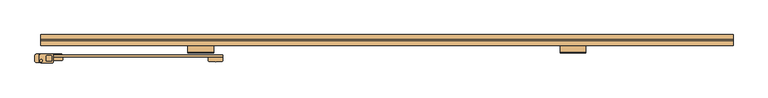
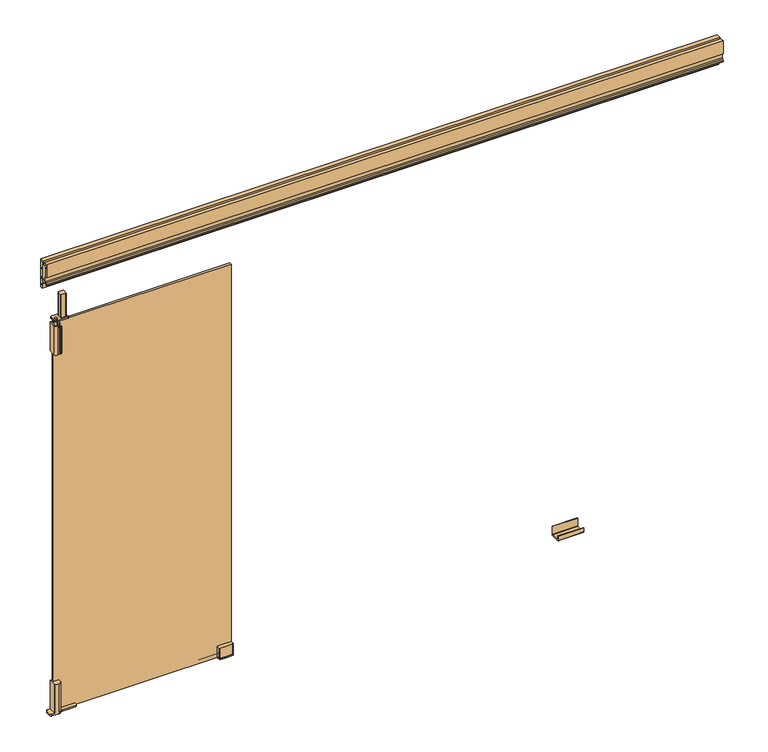
"""IFC4 building model written with IfcOpenShell, lengths in millimetres: door geometry, Otomatik Kapı-Tek Kanat : Otomatik Kapı - Tek Kanat."""

from ifc_helpers import new_model, si_unit, point, frame, frame_2d, origin, origin_with_axes, place, context, project, spatial, polyline, circle_curve, trimmed, segment, composite_curve, outline, extrude, source, transform, mapped, element, save
from ifc_brep_helpers import plane_surface, cylinder_surface, revolved_surface, advanced_brep


def door_8b1a0773(model_context):
    return source(origin(), model_context, "Body", "SolidModel", [
        advanced_brep(
        [(-1574.3473639, -189.1450647, 150.5), (-1574.3473639, -187.0776187, 150.5), (-1576.2799178, -185.1450647, 150.5), (-1605.0612263, -185.1450647, 150.5), (-1606.9937802, -187.0776187, 150.5), (-1606.9937802, -222.3613608, 150.5), (-1605.2100763, -224.1450647, 150.5), (-1587.4005623, -224.1450647, 150.5), (-1574.9937802, -217.3610561, 150.5), (-1574.9937802, -199.1283088, 150.5), (-1599.9937802, -199.1283088, 150.5), (-1599.9937802, -189.1450647, 150.5), (-1578.9203726, -221.1098306, 8.0), (-1577.1630779, -219.3712473, 8.0), (-1574.9937802, -217.3610561, 8.0), (-1599.9937802, -189.1450647, 8.0), (-1574.3473639, -189.1450647, 8.0), (-1599.9937802, -199.1283088, 8.0), (-1574.9937802, -199.1283088, 8.0), (-1587.4005623, -224.1450647, 8.0), (-1605.2100763, -224.1450647, 8.0), (-1619.8416735, -224.1450647, 8.0), (-1619.8416735, -224.1450647, 0.0), (-1587.4005623, -224.1450647, 0.0), (-1606.9937802, -222.3613608, 8.0), (-1606.9937802, -187.0776187, 8.0), (-1605.0612263, -185.1450647, 8.0), (-1576.2799178, -185.1450647, 8.0), (-1504.0, -185.1450647, 8.0), (-1504.0, -185.1450647, 0.0), (-1619.9440671, -185.1450647, 0.0), (-1619.9440671, -185.1450647, 8.0), (-1574.3473639, -187.0776187, 8.0), (-1499.0, -190.1450647, 0.0), (-1499.0, -210.1450647, 0.0), (-1504.0, -215.1450647, 0.0), (-1568.1, -215.1450647, 0.0), (-1577.1630779, -219.3712473, 0.0), (-1627.0, -216.9867382, 0.0), (-1627.0, -192.2009976, 0.0), (-1627.0, -192.2009976, 8.0), (-1627.0, -216.9867382, 8.0), (-1568.1, -215.1450647, 8.0), (-1504.0, -215.1450647, 8.0), (-1499.0, -210.1450647, 8.0), (-1499.0, -190.1450647, 8.0)],
        [
            (0, 1),
            (1, 2, circle_curve(frame((-1576.2799178, -187.0776187, 150.5), z_axis=(0.0, 0.0, 1.0), x_axis=(1.0, 0.0, 0.0)), 1.932554)),
            (2, 3),
            (3, 4, circle_curve(frame((-1605.0612263, -187.0776187, 150.5), z_axis=(0.0, 0.0, 1.0), x_axis=(1.0, 0.0, 0.0)), 1.932554)),
            (4, 5),
            (5, 6, circle_curve(frame((-1605.2100763, -222.3613608, 150.5), z_axis=(0.0, 0.0, 1.0), x_axis=(1.0, 0.0, 0.0)), 1.7837039)),
            (6, 7),
            (7, 8, circle_curve(frame((-1588.8230743, -206.8065986, 150.5), z_axis=(0.0, 0.0, 1.0), x_axis=(1.0, 0.0, 0.0)), 17.3967223)),
            (8, 9),
            (9, 10),
            (10, 11),
            (11, 0),
            (12, 13, circle_curve(frame((-1587.4005623, -210.7809779, 8.0), z_axis=(0.0, 0.0, 1.0), x_axis=(1.0, 0.0, 0.0)), 13.3640868)),
            (13, 14, circle_curve(frame((-1568.1, -226.9760726, 8.0), z_axis=(0.0, 0.0, -1.0), x_axis=(1.0, 0.0, 0.0)), 11.8310079)),
            (14, 12, circle_curve(frame((-1588.8230743, -206.8065986, 8.0), z_axis=(0.0, 0.0, -1.0), x_axis=(1.0, 0.0, 0.0)), 17.3967223)),
            (11, 15),
            (15, 16),
            (16, 0),
            (10, 17),
            (17, 15),
            (9, 18),
            (18, 17),
            (8, 14),
            (14, 18),
            (7, 19),
            (19, 12, circle_curve(frame((-1588.8230743, -206.8065986, 8.0), z_axis=(0.0, 0.0, 1.0), x_axis=(1.0, 0.0, 0.0)), 17.3967223)),
            (6, 20),
            (20, 21),
            (21, 22),
            (22, 23),
            (23, 19),
            (5, 24),
            (24, 20, circle_curve(frame((-1605.2100763, -222.3613608, 8.0), z_axis=(0.0, 0.0, 1.0), x_axis=(1.0, 0.0, 0.0)), 1.7837039)),
            (4, 25),
            (25, 24),
            (3, 26),
            (26, 25, circle_curve(frame((-1605.0612263, -187.0776187, 8.0), z_axis=(0.0, 0.0, 1.0), x_axis=(1.0, 0.0, 0.0)), 1.932554)),
            (2, 27),
            (27, 28),
            (28, 29),
            (29, 30),
            (30, 31),
            (31, 26),
            (1, 32),
            (32, 27, circle_curve(frame((-1576.2799178, -187.0776187, 8.0), z_axis=(0.0, 0.0, 1.0), x_axis=(1.0, 0.0, 0.0)), 1.932554)),
            (16, 32),
            (29, 33, circle_curve(frame((-1504.0, -190.1450647, 0.0), z_axis=(0.0, 0.0, -1.0), x_axis=(1.0, 0.0, 0.0)), 5.0)),
            (33, 34),
            (34, 35, circle_curve(frame((-1504.0, -210.1450647, 0.0), z_axis=(0.0, 0.0, -1.0), x_axis=(1.0, 0.0, 0.0)), 5.0)),
            (35, 36),
            (36, 37, circle_curve(frame((-1568.1, -226.9760726, 0.0), z_axis=(0.0, 0.0, 1.0), x_axis=(1.0, 0.0, 0.0)), 11.8310079)),
            (37, 23, circle_curve(frame((-1587.4005623, -210.7809779, 0.0), z_axis=(0.0, 0.0, -1.0), x_axis=(1.0, 0.0, 0.0)), 13.3640868)),
            (22, 38, circle_curve(frame((-1619.8416735, -216.9867382, 0.0), z_axis=(0.0, 0.0, -1.0), x_axis=(1.0, 0.0, 0.0)), 7.1583265)),
            (38, 39),
            (39, 30, circle_curve(frame((-1619.9440671, -192.2009976, 0.0), z_axis=(0.0, 0.0, -1.0), x_axis=(1.0, 0.0, 0.0)), 7.0559329)),
            (19, 12, circle_curve(frame((-1587.4005623, -210.7809779, 8.0), z_axis=(0.0, 0.0, 1.0), x_axis=(1.0, 0.0, 0.0)), 13.3640868)),
            (31, 40, circle_curve(frame((-1619.9440671, -192.2009976, 8.0), z_axis=(0.0, 0.0, 1.0), x_axis=(1.0, 0.0, 0.0)), 7.0559329)),
            (40, 41),
            (41, 21, circle_curve(frame((-1619.8416735, -216.9867382, 8.0), z_axis=(0.0, 0.0, 1.0), x_axis=(1.0, 0.0, 0.0)), 7.1583265)),
            (14, 42, circle_curve(frame((-1568.1, -226.9760726, 8.0), z_axis=(0.0, 0.0, -1.0), x_axis=(1.0, 0.0, 0.0)), 11.8310079)),
            (42, 43),
            (43, 44, circle_curve(frame((-1504.0, -210.1450647, 8.0), z_axis=(0.0, 0.0, 1.0), x_axis=(1.0, 0.0, 0.0)), 5.0)),
            (44, 45),
            (45, 28, circle_curve(frame((-1504.0, -190.1450647, 8.0), z_axis=(0.0, 0.0, 1.0), x_axis=(1.0, 0.0, 0.0)), 5.0)),
            (39, 40),
            (38, 41),
            (37, 13),
            (36, 42),
            (35, 43),
            (34, 44),
            (33, 45),
        ],
        [
            plane_surface(frame((-1627.0, -185.1450647, 150.5), z_axis=(0.0, 0.0, 1.0), x_axis=(0.0, 1.0, 0.0))),
            plane_surface(frame((-1627.0, -185.1450647, 8.0), z_axis=(0.0, 0.0, -1.0), x_axis=(0.0, 1.0, 0.0))),
            plane_surface(frame((-1574.3473639, -189.1450647, 150.5), z_axis=(0.0, -1.0, 0.0), x_axis=(0.0, 0.0, -1.0))),
            plane_surface(frame((-1599.9937802, -189.1450647, 150.5), z_axis=(1.0, 0.0, 0.0), x_axis=(0.0, 0.0, -1.0))),
            plane_surface(frame((-1599.9937802, -199.1283088, 150.5), z_axis=(0.0, 1.0, 0.0), x_axis=(0.0, 0.0, -1.0))),
            plane_surface(frame((-1574.9937802, -199.1283088, 150.5), z_axis=(1.0, 0.0, 0.0), x_axis=(0.0, 0.0, -1.0))),
            cylinder_surface(frame((-1588.8230743, -206.8065986, 150.5), z_axis=(0.0, 0.0, 1.0), x_axis=(1.0, 0.0, 0.0)), 17.3967223),
            plane_surface(frame((-1587.4005623, -224.1450647, 150.5), z_axis=(0.0, -1.0, 0.0), x_axis=(0.0, 0.0, -1.0))),
            cylinder_surface(frame((-1605.2100763, -222.3613608, 150.5), z_axis=(0.0, 0.0, 1.0), x_axis=(1.0, 0.0, 0.0)), 1.7837039),
            plane_surface(frame((-1606.9937802, -222.3613608, 150.5), z_axis=(-1.0, 0.0, 0.0), x_axis=(0.0, 0.0, -1.0))),
            cylinder_surface(frame((-1605.0612263, -187.0776187, 150.5), z_axis=(0.0, 0.0, 1.0), x_axis=(1.0, 0.0, 0.0)), 1.932554),
            plane_surface(frame((-1605.0612263, -185.1450647, 150.5), z_axis=(0.0, 1.0, 0.0), x_axis=(0.0, 0.0, -1.0))),
            cylinder_surface(frame((-1576.2799178, -187.0776187, 150.5), z_axis=(0.0, 0.0, 1.0), x_axis=(1.0, 0.0, 0.0)), 1.932554),
            plane_surface(frame((-1574.3473639, -187.0776187, 150.5), z_axis=(1.0, 0.0, 0.0), x_axis=(0.0, 0.0, -1.0))),
            plane_surface(frame((-1627.0, -185.1450647, 0.0), z_axis=(0.0, 0.0, -1.0), x_axis=(0.0, 1.0, 0.0))),
            plane_surface(frame((-1627.0, -185.1450647, 8.0), z_axis=(0.0, 0.0, 1.0), x_axis=(0.0, 1.0, 0.0))),
            cylinder_surface(frame((-1619.9440671, -192.2009976, 0.0), z_axis=(0.0, 0.0, -1.0), x_axis=(1.0, 0.0, 0.0)), 7.0559329),
            plane_surface(frame((-1627.0, -192.2009976, 0.0), z_axis=(-1.0, 0.0, 0.0), x_axis=(0.0, 0.0, 1.0))),
            cylinder_surface(frame((-1619.8416735, -216.9867382, 0.0), z_axis=(0.0, 0.0, -1.0), x_axis=(1.0, 0.0, 0.0)), 7.1583265),
            cylinder_surface(frame((-1587.4005623, -210.7809779, 0.0), z_axis=(0.0, 0.0, -1.0), x_axis=(1.0, 0.0, 0.0)), 13.3640868),
            revolved_surface(polyline([(-1556.2689920999999, -226.9760726, 8.0), (-1556.2689920999999, -226.9760726, 0.0)]), (-1568.1, -226.9760726, 0.0), (0.0, 0.0, 1.0)),
            plane_surface(frame((-1568.1, -215.1450647, 0.0), z_axis=(0.0, -1.0, 0.0), x_axis=(0.0, 0.0, 1.0))),
            cylinder_surface(frame((-1504.0, -210.1450647, 0.0), z_axis=(0.0, 0.0, -1.0), x_axis=(1.0, 0.0, 0.0)), 5.0),
            plane_surface(frame((-1499.0, -210.1450647, 0.0), z_axis=(1.0, 0.0, 0.0), x_axis=(0.0, 0.0, 1.0))),
            cylinder_surface(frame((-1504.0, -190.1450647, 0.0), z_axis=(0.0, 0.0, -1.0), x_axis=(1.0, 0.0, 0.0)), 5.0),
        ],
        [
            (0, [[1, 2, 3, 4, 5, 6, 7, 8, 9, 10, 11, 12]]),
            (1, [[13, 14, 15]]),
            (2, [[16, 17, 18, -12]]),
            (3, [[19, 20, -16, -11]]),
            (4, [[21, 22, -19, -10]]),
            (5, [[23, 24, -21, -9]]),
            (6, [[25, 26, -15, -23, -8]]),
            (7, [[27, 28, 29, 30, 31, -25, -7]]),
            (8, [[32, 33, -27, -6]]),
            (9, [[34, 35, -32, -5]]),
            (10, [[36, 37, -34, -4]]),
            (11, [[38, 39, 40, 41, 42, 43, -36, -3]]),
            (12, [[44, 45, -38, -2]]),
            (13, [[-18, 46, -44, -1]]),
            (14, [[47, 48, 49, 50, 51, 52, -30, 53, 54, 55, -41]]),
            (15, [[-26, 56]]),
            (15, [[-28, -33, -35, -37, -43, 57, 58, 59]]),
            (15, [[-39, -45, -46, -17, -20, -22, -24, 60, 61, 62, 63, 64]]),
            (16, [[65, -57, -42, -55]]),
            (17, [[66, -58, -65, -54]]),
            (18, [[-29, -59, -66, -53]]),
            (19, [[67, -13, -56, -31, -52]]),
            (20, [[68, -60, -14, -67, -51]]),
            (21, [[69, -61, -68, -50]]),
            (22, [[70, -62, -69, -49]]),
            (23, [[71, -63, -70, -48]]),
            (24, [[-40, -64, -71, -47]]),
        ],
    ),
        advanced_brep(
        [(-1572.1438552, -192.4241594, 2085.0), (-1573.9791404, -194.2594446, 2085.0), (-1573.9791404, -215.5888742, 2085.0), (-1572.1438552, -217.4241594, 2085.0), (-1550.8144257, -217.4241594, 2085.0), (-1548.9791404, -215.5888742, 2085.0), (-1548.9791404, -194.2594446, 2085.0), (-1550.8144257, -192.4241594, 2085.0), (-1550.8144257, -192.4241594, 1970.0), (-1572.1438552, -192.4241594, 1970.0), (-1548.9791404, -194.2594446, 1970.0), (-1548.9791404, -215.5888742, 1970.0), (-1550.8144257, -217.4241594, 1970.0), (-1572.1438552, -217.4241594, 1970.0), (-1573.9791404, -215.5888742, 1970.0), (-1573.9791404, -194.2594446, 1970.0), (-1545.9964024, -185.1450647, 1970.0), (-1598.1649399, -185.1450647, 1970.0), (-1606.9937802, -193.9739051, 1970.0), (-1606.9937802, -216.1450647, 1970.0), (-1597.9937802, -225.1450647, 1970.0), (-1546.3153559, -225.1450647, 1970.0), (-1542.9937802, -221.823489, 1970.0), (-1542.9937802, -188.1476868, 1970.0), (-1597.9937802, -222.0450647, 1970.0), (-1597.9937802, -210.2450647, 1970.0), (-1545.9964024, -185.1450647, 1964.0), (-1542.9937802, -188.1476868, 1964.0), (-1542.9937802, -221.823489, 1964.0), (-1546.3153559, -225.1450647, 1964.0), (-1597.9937802, -225.1450647, 1964.0), (-1606.9937802, -216.1450647, 1964.0), (-1606.9937802, -193.9739051, 1964.0), (-1598.1649399, -185.1450647, 1964.0), (-1597.9937802, -210.2450647, 1964.0), (-1597.9937802, -222.0450647, 1964.0), (-1606.9937802, -216.1450647, 1798.2), (-1606.9937802, -186.3566653, 1798.2), (-1605.7821796, -185.1450647, 1798.2), (-1576.3197681, -185.1450647, 1798.2), (-1574.9937802, -186.4710526, 1798.2), (-1574.9937802, -189.2450647, 1798.2), (-1599.7937802, -189.2450647, 1798.2), (-1599.7937802, -199.2450647, 1798.2), (-1574.9937802, -199.2450647, 1798.2), (-1574.9937802, -222.0450647, 1798.2), (-1578.0937802, -225.1450647, 1798.2), (-1587.411505, -225.1450647, 1798.2), (-1591.4461955, -222.319944, 1798.2), (-1587.2194224, -210.2450647, 1798.2), (-1588.9937802, -212.0194225, 1798.2), (-1588.9937802, -219.8725331, 1798.2), (-1587.1673699, -222.0450647, 1798.2), (-1579.0825581, -222.0450647, 1798.2), (-1578.0937802, -221.0562868, 1798.2), (-1578.0937802, -210.2450647, 1798.2), (-1597.9937802, -210.2450647, 1798.2), (-1597.9937802, -222.0450647, 1798.2), (-1606.9937802, -216.1450647, 1943.2), (-1588.9937802, -216.1450647, 1943.2), (-1588.9937802, -212.0194225, 1943.2), (-1587.2194224, -210.2450647, 1943.2), (-1576.1717604, -210.2450647, 1943.2), (-1574.9937802, -209.0670845, 1943.2), (-1574.9937802, -199.2450647, 1943.2), (-1599.7937802, -199.2450647, 1943.2), (-1599.7937802, -189.2450647, 1943.2), (-1574.9937802, -189.2450647, 1943.2), (-1574.9937802, -186.4710526, 1943.2), (-1576.3197681, -185.1450647, 1943.2), (-1605.7821796, -185.1450647, 1943.2), (-1606.9937802, -186.3566653, 1943.2), (-1597.9937802, -222.0450647, 1943.2), (-1597.9937802, -210.2450647, 1943.2), (-1574.9937802, -209.0670845, 1933.2), (-1574.9937802, -222.0450647, 1933.2), (-1576.1717604, -210.2450647, 1933.2), (-1578.0937802, -210.2450647, 1933.2), (-1588.9937802, -216.1450647, 1933.2), (-1588.9937802, -219.8725331, 1933.2), (-1591.4461955, -222.319944, 1933.2), (-1597.9937802, -210.2450647, 1943.2), (-1597.9937802, -222.0450647, 1943.2), (-1578.0937802, -225.1450647, 1933.2), (-1578.0937802, -221.0562868, 1933.2), (-1579.0825581, -222.0450647, 1933.2), (-1587.1673699, -222.0450647, 1933.2), (-1587.411505, -225.1450647, 1933.2), (-1597.9937802, -210.2450647, 1976.5286826), (-1597.9937802, -222.0450647, 1976.5286826)],
        [
            (0, 1, circle_curve(frame((-1572.1438552, -194.2594446, 2085.0), z_axis=(0.0, 0.0, 1.0), x_axis=(0.0, -1.0, 0.0)), 1.8352852)),
            (1, 2),
            (2, 3, circle_curve(frame((-1572.1438552, -215.5888742, 2085.0), z_axis=(0.0, 0.0, 1.0), x_axis=(0.0, 1.0, 0.0)), 1.8352852)),
            (3, 4),
            (4, 5, circle_curve(frame((-1550.8144257, -215.5888742, 2085.0), z_axis=(0.0, 0.0, 1.0), x_axis=(0.0, 1.0, 0.0)), 1.8352852)),
            (5, 6),
            (6, 7, circle_curve(frame((-1550.8144257, -194.2594446, 2085.0), z_axis=(0.0, 0.0, 1.0), x_axis=(0.0, -1.0, 0.0)), 1.8352852)),
            (7, 0),
            (7, 8),
            (8, 9),
            (9, 0),
            (6, 10),
            (10, 8, circle_curve(frame((-1550.8144257, -194.2594446, 1970.0), z_axis=(0.0, 0.0, 1.0), x_axis=(0.0, -1.0, 0.0)), 1.8352852)),
            (5, 11),
            (11, 10),
            (4, 12),
            (12, 11, circle_curve(frame((-1550.8144257, -215.5888742, 1970.0), z_axis=(0.0, 0.0, 1.0), x_axis=(0.0, 1.0, 0.0)), 1.8352852)),
            (3, 13),
            (13, 12),
            (2, 14),
            (14, 13, circle_curve(frame((-1572.1438552, -215.5888742, 1970.0), z_axis=(0.0, 0.0, 1.0), x_axis=(0.0, 1.0, 0.0)), 1.8352852)),
            (1, 15),
            (15, 14),
            (9, 15, circle_curve(frame((-1572.1438552, -194.2594446, 1970.0), z_axis=(0.0, 0.0, 1.0), x_axis=(0.0, -1.0, 0.0)), 1.8352852)),
            (16, 17),
            (17, 18, circle_curve(frame((-1598.1649399, -193.9739051, 1970.0), z_axis=(0.0, 0.0, 1.0), x_axis=(0.0, -1.0, 0.0)), 8.8288404)),
            (18, 19),
            (19, 20, circle_curve(frame((-1597.9937802, -216.1450647, 1970.0), z_axis=(0.0, 0.0, 1.0), x_axis=(0.0, -1.0, 0.0)), 9.0)),
            (20, 21),
            (21, 22, circle_curve(frame((-1546.3153559, -221.823489, 1970.0), z_axis=(0.0, 0.0, 1.0), x_axis=(0.0, -1.0, 0.0)), 3.3215757)),
            (22, 23),
            (23, 16, circle_curve(frame((-1545.9964024, -188.1476868, 1970.0), z_axis=(0.0, 0.0, 1.0), x_axis=(0.0, -1.0, 0.0)), 3.0026222)),
            (24, 25, circle_curve(frame((-1597.9937802, -216.1450647, 1970.0), z_axis=(0.0, 0.0, -1.0), x_axis=(0.0, -1.0, 0.0)), 5.9)),
            (25, 24, circle_curve(frame((-1597.9937802, -216.1450647, 1970.0), z_axis=(0.0, 0.0, -1.0), x_axis=(0.0, -1.0, 0.0)), 5.9)),
            (26, 27, circle_curve(frame((-1545.9964024, -188.1476868, 1964.0), z_axis=(0.0, 0.0, -1.0), x_axis=(0.0, -1.0, 0.0)), 3.0026222)),
            (27, 28),
            (28, 29, circle_curve(frame((-1546.3153559, -221.823489, 1964.0), z_axis=(0.0, 0.0, -1.0), x_axis=(0.0, -1.0, 0.0)), 3.3215757)),
            (29, 30),
            (30, 31, circle_curve(frame((-1597.9937802, -216.1450647, 1964.0), z_axis=(0.0, 0.0, -1.0), x_axis=(0.0, -1.0, 0.0)), 9.0)),
            (31, 32),
            (32, 33, circle_curve(frame((-1598.1649399, -193.9739051, 1964.0), z_axis=(0.0, 0.0, -1.0), x_axis=(0.0, -1.0, 0.0)), 8.8288404)),
            (33, 26),
            (34, 35, circle_curve(frame((-1597.9937802, -216.1450647, 1964.0), z_axis=(0.0, 0.0, 1.0), x_axis=(0.0, -1.0, 0.0)), 5.9)),
            (35, 34, circle_curve(frame((-1597.9937802, -216.1450647, 1964.0), z_axis=(0.0, 0.0, 1.0), x_axis=(0.0, -1.0, 0.0)), 5.9)),
            (16, 26),
            (33, 17),
            (32, 18),
            (31, 19),
            (30, 20),
            (29, 21),
            (28, 22),
            (27, 23),
            (36, 37),
            (37, 38, circle_curve(frame((-1605.7821796, -186.3566653, 1798.2), z_axis=(0.0, 0.0, -1.0), x_axis=(0.0, -1.0, 0.0)), 1.2116006)),
            (38, 39),
            (39, 40, circle_curve(frame((-1576.3197681, -186.4710526, 1798.2), z_axis=(0.0, 0.0, -1.0), x_axis=(0.0, -1.0, 0.0)), 1.3259879)),
            (40, 41),
            (41, 42),
            (42, 43),
            (43, 44),
            (44, 45),
            (45, 46, circle_curve(frame((-1578.0937802, -222.0450647, 1798.2), z_axis=(0.0, 0.0, -1.0), x_axis=(0.0, -1.0, 0.0)), 3.1)),
            (46, 47),
            (47, 48, circle_curve(frame((-1586.7260693, -219.8725331, 1798.2), z_axis=(0.0, 0.0, -1.0), x_axis=(0.0, -1.0, 0.0)), 5.3168987)),
            (48, 36, circle_curve(frame((-1597.9937802, -216.1450647, 1798.2), z_axis=(0.0, 0.0, -1.0), x_axis=(0.0, -1.0, 0.0)), 9.0)),
            (49, 50, circle_curve(frame((-1587.2194224, -212.0194225, 1798.2), z_axis=(0.0, 0.0, 1.0), x_axis=(0.0, -1.0, 0.0)), 1.7743579)),
            (50, 51),
            (51, 52, circle_curve(frame((-1586.7260693, -219.8725331, 1798.2), z_axis=(0.0, 0.0, 1.0), x_axis=(0.0, -1.0, 0.0)), 2.2168987)),
            (52, 53),
            (53, 54, circle_curve(frame((-1579.0825581, -221.0562868, 1798.2), z_axis=(0.0, 0.0, 1.0), x_axis=(0.0, -1.0, 0.0)), 0.9887779)),
            (54, 55),
            (55, 49),
            (56, 57, circle_curve(frame((-1597.9937802, -216.1450647, 1798.2), z_axis=(0.0, 0.0, 1.0), x_axis=(0.0, -1.0, 0.0)), 5.9)),
            (57, 56, circle_curve(frame((-1597.9937802, -216.1450647, 1798.2), z_axis=(0.0, 0.0, 1.0), x_axis=(0.0, -1.0, 0.0)), 5.9)),
            (58, 59, circle_curve(frame((-1597.9937802, -216.1450647, 1943.2), z_axis=(0.0, 0.0, 1.0), x_axis=(0.0, -1.0, 0.0)), 9.0)),
            (59, 60),
            (60, 61, circle_curve(frame((-1587.2194224, -212.0194225, 1943.2), z_axis=(0.0, 0.0, -1.0), x_axis=(0.0, -1.0, 0.0)), 1.7743579)),
            (61, 62),
            (62, 63, circle_curve(frame((-1576.1717604, -209.0670845, 1943.2), z_axis=(0.0, 0.0, 1.0), x_axis=(0.0, -1.0, 0.0)), 1.1779802)),
            (63, 64),
            (64, 65),
            (65, 66),
            (66, 67),
            (67, 68),
            (68, 69, circle_curve(frame((-1576.3197681, -186.4710526, 1943.2), z_axis=(0.0, 0.0, 1.0), x_axis=(0.0, -1.0, 0.0)), 1.3259879)),
            (69, 70),
            (70, 71, circle_curve(frame((-1605.7821796, -186.3566653, 1943.2), z_axis=(0.0, 0.0, 1.0), x_axis=(0.0, -1.0, 0.0)), 1.2116006)),
            (71, 58),
            (72, 73, circle_curve(frame((-1597.9937802, -216.1450647, 1943.2), z_axis=(0.0, 0.0, -1.0), x_axis=(0.0, -1.0, 0.0)), 5.9)),
            (73, 72, circle_curve(frame((-1597.9937802, -216.1450647, 1943.2), z_axis=(0.0, 0.0, -1.0), x_axis=(0.0, -1.0, 0.0)), 5.9)),
            (36, 58),
            (71, 37),
            (70, 38),
            (69, 39),
            (68, 40),
            (67, 41),
            (66, 42),
            (65, 43),
            (64, 44),
            (63, 74),
            (74, 75),
            (75, 45),
            (62, 76),
            (76, 74, circle_curve(frame((-1576.1717604, -209.0670845, 1933.2), z_axis=(0.0, 0.0, 1.0), x_axis=(0.0, -1.0, 0.0)), 1.1779802)),
            (61, 49),
            (55, 77),
            (77, 76),
            (60, 50),
            (59, 78),
            (78, 79),
            (79, 51),
            (48, 80),
            (80, 78, circle_curve(frame((-1597.9937802, -216.1450647, 1933.2), z_axis=(0.0, 0.0, 1.0), x_axis=(0.0, -1.0, 0.0)), 9.0)),
            (56, 81),
            (81, 82, circle_curve(frame((-1597.9937802, -216.1450647, 1943.2), z_axis=(0.0, 0.0, 1.0), x_axis=(0.0, -1.0, 0.0)), 5.9)),
            (82, 57),
            (82, 81, circle_curve(frame((-1597.9937802, -216.1450647, 1943.2), z_axis=(0.0, 0.0, 1.0), x_axis=(0.0, -1.0, 0.0)), 5.9)),
            (83, 75, circle_curve(frame((-1578.0937802, -222.0450647, 1933.2), z_axis=(0.0, 0.0, 1.0), x_axis=(0.0, -1.0, 0.0)), 3.1)),
            (77, 84),
            (84, 85, circle_curve(frame((-1579.0825581, -221.0562868, 1933.2), z_axis=(0.0, 0.0, -1.0), x_axis=(0.0, -1.0, 0.0)), 0.9887779)),
            (85, 86),
            (86, 79, circle_curve(frame((-1586.7260693, -219.8725331, 1933.2), z_axis=(0.0, 0.0, -1.0), x_axis=(0.0, -1.0, 0.0)), 2.2168987)),
            (80, 87, circle_curve(frame((-1586.7260693, -219.8725331, 1933.2), z_axis=(0.0, 0.0, 1.0), x_axis=(0.0, -1.0, 0.0)), 5.3168987)),
            (87, 83),
            (83, 46),
            (54, 84),
            (53, 85),
            (52, 86),
            (47, 87),
            (88, 89, circle_curve(frame((-1597.9937802, -216.1450647, 1976.5286826), z_axis=(0.0, 0.0, 1.0), x_axis=(0.0, -1.0, 0.0)), 5.9)),
            (89, 88, circle_curve(frame((-1597.9937802, -216.1450647, 1976.5286826), z_axis=(0.0, 0.0, 1.0), x_axis=(0.0, -1.0, 0.0)), 5.9)),
            (88, 25),
            (24, 89),
            (34, 73),
            (72, 35),
        ],
        [
            plane_surface(frame((-1606.9937802, -185.1450647, 2085.0), z_axis=(0.0, 0.0, 1.0), x_axis=(-1.0, 0.0, 0.0))),
            plane_surface(frame((-1572.1438552, -192.4241594, 1970.0), z_axis=(0.0, 1.0, 0.0), x_axis=(0.0, 0.0, 1.0))),
            cylinder_surface(frame((-1550.8144257, -194.2594446, 1970.0), z_axis=(0.0, 0.0, -1.0), x_axis=(0.0, -1.0, 0.0)), 1.8352852),
            plane_surface(frame((-1548.9791404, -194.2594446, 1970.0), z_axis=(1.0, 0.0, 0.0), x_axis=(0.0, 0.0, 1.0))),
            cylinder_surface(frame((-1550.8144257, -215.5888742, 1970.0), z_axis=(0.0, 0.0, -1.0), x_axis=(0.0, 1.0, 0.0)), 1.8352852),
            plane_surface(frame((-1550.8144257, -217.4241594, 1970.0), z_axis=(0.0, -1.0, 0.0), x_axis=(0.0, 0.0, 1.0))),
            cylinder_surface(frame((-1572.1438552, -215.5888742, 1970.0), z_axis=(0.0, 0.0, -1.0), x_axis=(0.0, 1.0, 0.0)), 1.8352852),
            plane_surface(frame((-1573.9791404, -215.5888742, 1970.0), z_axis=(-1.0, 0.0, 0.0), x_axis=(0.0, 0.0, 1.0))),
            cylinder_surface(frame((-1572.1438552, -194.2594446, 1970.0), z_axis=(0.0, 0.0, -1.0), x_axis=(0.0, -1.0, 0.0)), 1.8352852),
            plane_surface(frame((-1606.9937802, -185.1450647, 1970.0), z_axis=(0.0, 0.0, 1.0), x_axis=(-1.0, 0.0, 0.0))),
            plane_surface(frame((-1606.9937802, -185.1450647, 1964.0), z_axis=(0.0, 0.0, -1.0), x_axis=(-1.0, 0.0, 0.0))),
            plane_surface(frame((-1545.9964024, -185.1450647, 1970.0), z_axis=(0.0, 1.0, 0.0), x_axis=(0.0, 0.0, -1.0))),
            cylinder_surface(frame((-1598.1649399, -193.9739051, 1970.0), z_axis=(0.0, 0.0, 1.0), x_axis=(0.0, -1.0, 0.0)), 8.8288404),
            plane_surface(frame((-1606.9937802, -193.9739051, 1970.0), z_axis=(-1.0, 0.0, 0.0), x_axis=(0.0, 0.0, -1.0))),
            cylinder_surface(frame((-1597.9937802, -216.1450647, 1970.0), z_axis=(0.0, 0.0, 1.0), x_axis=(0.0, -1.0, 0.0)), 9.0),
            plane_surface(frame((-1597.9937802, -225.1450647, 1970.0), z_axis=(0.0, -1.0, 0.0), x_axis=(0.0, 0.0, -1.0))),
            cylinder_surface(frame((-1546.3153559, -221.823489, 1970.0), z_axis=(0.0, 0.0, 1.0), x_axis=(0.0, -1.0, 0.0)), 3.3215757),
            plane_surface(frame((-1542.9937802, -221.823489, 1970.0), z_axis=(1.0, 0.0, 0.0), x_axis=(0.0, 0.0, -1.0))),
            cylinder_surface(frame((-1545.9964024, -188.1476868, 1970.0), z_axis=(0.0, 0.0, 1.0), x_axis=(0.0, -1.0, 0.0)), 3.0026222),
            plane_surface(frame((-1606.9937802, -185.1450647, 1798.2), z_axis=(0.0, 0.0, -1.0), x_axis=(-1.0, 0.0, 0.0))),
            plane_surface(frame((-1606.9937802, -185.1450647, 1943.2), z_axis=(0.0, 0.0, 1.0), x_axis=(-1.0, 0.0, 0.0))),
            plane_surface(frame((-1606.9937802, -216.1450647, 1798.2), z_axis=(-1.0, 0.0, 0.0), x_axis=(0.0, 0.0, 1.0))),
            cylinder_surface(frame((-1605.7821796, -186.3566653, 1798.2), z_axis=(0.0, 0.0, -1.0), x_axis=(0.0, -1.0, 0.0)), 1.2116006),
            plane_surface(frame((-1605.7821796, -185.1450647, 1798.2), z_axis=(0.0, 1.0, 0.0), x_axis=(0.0, 0.0, 1.0))),
            cylinder_surface(frame((-1576.3197681, -186.4710526, 1798.2), z_axis=(0.0, 0.0, -1.0), x_axis=(0.0, -1.0, 0.0)), 1.3259879),
            plane_surface(frame((-1574.9937802, -186.4710526, 1798.2), z_axis=(1.0, 0.0, 0.0), x_axis=(0.0, 0.0, 1.0))),
            plane_surface(frame((-1574.9937802, -189.2450647, 1798.2), z_axis=(0.0, -1.0, 0.0), x_axis=(0.0, 0.0, 1.0))),
            plane_surface(frame((-1599.7937802, -189.2450647, 1798.2), z_axis=(1.0, 0.0, 0.0), x_axis=(0.0, 0.0, 1.0))),
            plane_surface(frame((-1599.7937802, -199.2450647, 1798.2), z_axis=(0.0, 1.0, 0.0), x_axis=(0.0, 0.0, 1.0))),
            plane_surface(frame((-1574.9937802, -199.2450647, 1798.2), z_axis=(1.0, 0.0, 0.0), x_axis=(0.0, 0.0, 1.0))),
            cylinder_surface(frame((-1576.1717604, -209.0670845, 1798.2), z_axis=(0.0, 0.0, -1.0), x_axis=(0.0, -1.0, 0.0)), 1.1779802),
            plane_surface(frame((-1576.1717604, -210.2450647, 1798.2), z_axis=(0.0, -1.0, 0.0), x_axis=(0.0, 0.0, 1.0))),
            revolved_surface(polyline([(-1587.2194224, -213.7937804, 1943.2), (-1587.2194224, -213.7937804, 1798.2)]), (-1587.2194224, -212.0194225, 1798.2), (0.0, 0.0, 1.0)),
            plane_surface(frame((-1588.9937802, -212.0194225, 1798.2), z_axis=(1.0, 0.0, 0.0), x_axis=(0.0, 0.0, 1.0))),
            cylinder_surface(frame((-1597.9937802, -216.1450647, 1798.2), z_axis=(0.0, 0.0, -1.0), x_axis=(0.0, -1.0, 0.0)), 9.0),
            revolved_surface(polyline([(-1597.9937802, -222.0450647, 1943.2), (-1597.9937802, -222.0450647, 1798.2)]), (-1597.9937802, -216.1450647, 1798.2), (0.0, 0.0, 1.0)),
            plane_surface(frame((-1606.9937802, -185.1450647, 1933.2), z_axis=(0.0, 0.0, 1.0), x_axis=(-1.0, 0.0, 0.0))),
            cylinder_surface(frame((-1578.0937802, -222.0450647, 1933.2), z_axis=(0.0, 0.0, 1.0), x_axis=(0.0, -1.0, 0.0)), 3.1),
            plane_surface(frame((-1578.0937802, -210.2450647, 1933.2), z_axis=(-1.0, 0.0, 0.0), x_axis=(0.0, 0.0, -1.0))),
            revolved_surface(polyline([(-1579.0825581, -222.0450647, 1798.2), (-1579.0825581, -222.0450647, 1933.2)]), (-1579.0825581, -221.0562868, 1933.2), (0.0, 0.0, -1.0)),
            plane_surface(frame((-1579.0825581, -222.0450647, 1933.2), z_axis=(0.0, 1.0, 0.0), x_axis=(0.0, 0.0, -1.0))),
            revolved_surface(polyline([(-1586.7260693, -222.0894318, 1798.2), (-1586.7260693, -222.0894318, 1933.2)]), (-1586.7260693, -219.8725331, 1933.2), (0.0, 0.0, -1.0)),
            cylinder_surface(frame((-1586.7260693, -219.8725331, 1933.2), z_axis=(0.0, 0.0, 1.0), x_axis=(0.0, -1.0, 0.0)), 5.3168987),
            plane_surface(frame((-1587.411505, -225.1450647, 1933.2), z_axis=(0.0, -1.0, 0.0), x_axis=(0.0, 0.0, -1.0))),
            plane_surface(frame((-1606.9937802, -185.1450647, 1976.5286826), z_axis=(0.0, 0.0, 1.0), x_axis=(-1.0, 0.0, 0.0))),
            plane_surface(frame((-1606.9937802, -185.1450647, 1943.2), z_axis=(0.0, 0.0, -1.0), x_axis=(-1.0, 0.0, 0.0))),
            cylinder_surface(frame((-1597.9937802, -216.1450647, 1976.5286826), z_axis=(0.0, 0.0, 1.0), x_axis=(0.0, -1.0, 0.0)), 5.9),
        ],
        [
            (0, [[1, 2, 3, 4, 5, 6, 7, 8]]),
            (1, [[-8, 9, 10, 11]]),
            (2, [[-7, 12, 13, -9]]),
            (3, [[-6, 14, 15, -12]]),
            (4, [[-5, 16, 17, -14]]),
            (5, [[-4, 18, 19, -16]]),
            (6, [[-3, 20, 21, -18]]),
            (7, [[-2, 22, 23, -20]]),
            (8, [[-1, -11, 24, -22]]),
            (9, [[25, 26, 27, 28, 29, 30, 31, 32], [-10, -13, -15, -17, -19, -21, -23, -24], [33, 34]]),
            (10, [[35, 36, 37, 38, 39, 40, 41, 42], [43, 44]]),
            (11, [[-25, 45, -42, 46]]),
            (12, [[-26, -46, -41, 47]]),
            (13, [[-27, -47, -40, 48]]),
            (14, [[-28, -48, -39, 49]]),
            (15, [[-29, -49, -38, 50]]),
            (16, [[-30, -50, -37, 51]]),
            (17, [[-31, -51, -36, 52]]),
            (18, [[-32, -52, -35, -45]]),
            (19, [[53, 54, 55, 56, 57, 58, 59, 60, 61, 62, 63, 64, 65], [66, 67, 68, 69, 70, 71, 72], [73, 74]]),
            (20, [[75, 76, 77, 78, 79, 80, 81, 82, 83, 84, 85, 86, 87, 88], [89, 90]]),
            (21, [[-53, 91, -88, 92]]),
            (22, [[-54, -92, -87, 93]]),
            (23, [[-55, -93, -86, 94]]),
            (24, [[-56, -94, -85, 95]]),
            (25, [[-57, -95, -84, 96]]),
            (26, [[-58, -96, -83, 97]]),
            (27, [[-59, -97, -82, 98]]),
            (28, [[-60, -98, -81, 99]]),
            (29, [[-80, 100, 101, 102, -61, -99]]),
            (30, [[-79, 103, 104, -100]]),
            (31, [[-78, 105, -72, 106, 107, -103]]),
            (32, [[-66, -105, -77, 108]]),
            (33, [[-76, 109, 110, 111, -67, -108]]),
            (34, [[-75, -91, -65, 112, 113, -109]]),
            (35, [[-73, 114, 115, 116]]),
            (35, [[-74, -116, 117, -114]]),
            (36, [[118, -101, -104, -107, 119, 120, 121, 122, -110, -113, 123, 124]]),
            (37, [[-118, 125, -62, -102]]),
            (38, [[-119, -106, -71, 126]]),
            (39, [[-120, -126, -70, 127]]),
            (40, [[-121, -127, -69, 128]]),
            (41, [[-122, -128, -68, -111]]),
            (42, [[-123, -112, -64, 129]]),
            (43, [[-124, -129, -63, -125]]),
            (44, [[130, 131]]),
            (45, [[-115, -117]]),
            (46, [[-130, 132, -33, 133]]),
            (46, [[134, -89, 135, -43]]),
            (46, [[-131, -133, -34, -132]]),
            (46, [[-134, -44, -135, -90]]),
        ],
    ),
        advanced_brep(
        [(-823.070583, -218.6262224, 6.5), (-825.3, -216.3968054, 6.5), (-825.3, -201.4058429, 6.5), (-823.0392218, -199.1450647, 6.5), (-761.5607782, -199.1450647, 6.5), (-759.3, -201.4058429, 6.5), (-759.3, -216.3968054, 6.5), (-761.529417, -218.6262224, 6.5), (-789.4, -203.8013241, 6.5), (-795.2, -203.8013241, 6.5), (-795.2, -214.0013241, 6.5), (-789.4, -214.0013241, 6.5), (-823.070583, -218.6262224, 56.5), (-761.529417, -218.6262224, 56.5), (-759.3, -216.3968054, 56.5), (-759.3, -201.4058429, 56.5), (-761.5607782, -199.1450647, 56.5), (-823.0392218, -199.1450647, 56.5), (-825.3, -201.4058429, 56.5), (-825.3, -216.3968054, 56.5), (-789.4, -203.8013241, 4.0), (-795.2, -203.8013241, 4.0), (-795.2, -214.0013241, 4.0), (-789.4, -214.0013241, 4.0), (-823.0392218, -199.1450647, 0.0), (-761.5607782, -199.1450647, 0.0), (-759.3, -201.4058429, 0.0), (-759.3, -216.3968054, 0.0), (-761.529417, -218.6262224, 0.0), (-823.070583, -218.6262224, 0.0), (-825.3, -216.3968054, 0.0), (-825.3, -201.4058429, 0.0), (-823.0392218, -199.1450647, 4.0), (-825.3, -201.4058429, 4.0), (-825.3, -216.3968054, 4.0), (-823.070583, -218.6262224, 4.0), (-761.529417, -218.6262224, 4.0), (-759.3, -216.3968054, 4.0), (-759.3, -201.4058429, 4.0), (-761.5607782, -199.1450647, 4.0)],
        [
            (0, 1, circle_curve(frame((-821.6131495, -214.9393719, 6.5), z_axis=(0.0, 0.0, -1.0), x_axis=(-1.0, 0.0, 0.0)), 3.9644646)),
            (1, 2),
            (2, 3, circle_curve(frame((-823.0392218, -201.4058429, 6.5), z_axis=(0.0, 0.0, -1.0), x_axis=(1.0, 0.0, 0.0)), 2.2607782)),
            (3, 4),
            (4, 5, circle_curve(frame((-761.5607782, -201.4058429, 6.5), z_axis=(0.0, 0.0, -1.0), x_axis=(-1.0, 0.0, 0.0)), 2.2607782)),
            (5, 6),
            (6, 7, circle_curve(frame((-762.9868505, -214.9393719, 6.5), z_axis=(0.0, 0.0, -1.0), x_axis=(1.0, 0.0, 0.0)), 3.9644646)),
            (7, 0, circle_curve(frame((-792.3, -31.936444, 6.5), z_axis=(0.0, 0.0, -1.0), x_axis=(-1.0, 0.0, 0.0)), 189.2086207)),
            (8, 9),
            (9, 10, circle_curve(frame((-795.2, -208.9013241, 6.5), z_axis=(0.0, 0.0, 1.0), x_axis=(-1.0, 0.0, 0.0)), 5.1)),
            (10, 11),
            (11, 8, circle_curve(frame((-789.4, -208.9013241, 6.5), z_axis=(0.0, 0.0, 1.0), x_axis=(-1.0, 0.0, 0.0)), 5.1)),
            (12, 13, circle_curve(frame((-792.3, -31.936444, 56.5), z_axis=(0.0, 0.0, 1.0), x_axis=(-1.0, 0.0, 0.0)), 189.2086207)),
            (13, 14, circle_curve(frame((-762.9868505, -214.9393719, 56.5), z_axis=(0.0, 0.0, 1.0), x_axis=(1.0, 0.0, 0.0)), 3.9644646)),
            (14, 15),
            (15, 16, circle_curve(frame((-761.5607782, -201.4058429, 56.5), z_axis=(0.0, 0.0, 1.0), x_axis=(-1.0, 0.0, 0.0)), 2.2607782)),
            (16, 17),
            (17, 18, circle_curve(frame((-823.0392218, -201.4058429, 56.5), z_axis=(0.0, 0.0, 1.0), x_axis=(1.0, 0.0, 0.0)), 2.2607782)),
            (18, 19),
            (19, 12, circle_curve(frame((-821.6131495, -214.9393719, 56.5), z_axis=(0.0, 0.0, 1.0), x_axis=(-1.0, 0.0, 0.0)), 3.9644646)),
            (0, 12),
            (19, 1),
            (18, 2),
            (17, 3),
            (16, 4),
            (15, 5),
            (14, 6),
            (13, 7),
            (8, 20),
            (20, 21),
            (21, 9),
            (21, 22, circle_curve(frame((-795.2, -208.9013241, 4.0), z_axis=(0.0, 0.0, 1.0), x_axis=(-1.0, 0.0, 0.0)), 5.1)),
            (22, 10),
            (22, 23),
            (23, 11),
            (23, 20, circle_curve(frame((-789.4, -208.9013241, 4.0), z_axis=(0.0, 0.0, 1.0), x_axis=(-1.0, 0.0, 0.0)), 5.1)),
            (24, 25),
            (25, 26, circle_curve(frame((-761.5607782, -201.4058429, 0.0), z_axis=(0.0, 0.0, -1.0), x_axis=(-1.0, 0.0, 0.0)), 2.2607782)),
            (26, 27),
            (27, 28, circle_curve(frame((-762.9868505, -214.9393719, 0.0), z_axis=(0.0, 0.0, -1.0), x_axis=(1.0, 0.0, 0.0)), 3.9644646)),
            (28, 29, circle_curve(frame((-792.3, -31.936444, 0.0), z_axis=(0.0, 0.0, -1.0), x_axis=(-1.0, 0.0, 0.0)), 189.2086207)),
            (29, 30, circle_curve(frame((-821.6131495, -214.9393719, 0.0), z_axis=(0.0, 0.0, -1.0), x_axis=(-1.0, 0.0, 0.0)), 3.9644646)),
            (30, 31),
            (31, 24, circle_curve(frame((-823.0392218, -201.4058429, 0.0), z_axis=(0.0, 0.0, -1.0), x_axis=(1.0, 0.0, 0.0)), 2.2607782)),
            (32, 33, circle_curve(frame((-823.0392218, -201.4058429, 4.0), z_axis=(0.0, 0.0, 1.0), x_axis=(1.0, 0.0, 0.0)), 2.2607782)),
            (33, 34),
            (34, 35, circle_curve(frame((-821.6131495, -214.9393719, 4.0), z_axis=(0.0, 0.0, 1.0), x_axis=(-1.0, 0.0, 0.0)), 3.9644646)),
            (35, 36, circle_curve(frame((-792.3, -31.936444, 4.0), z_axis=(0.0, 0.0, 1.0), x_axis=(-1.0, 0.0, 0.0)), 189.2086207)),
            (36, 37, circle_curve(frame((-762.9868505, -214.9393719, 4.0), z_axis=(0.0, 0.0, 1.0), x_axis=(1.0, 0.0, 0.0)), 3.9644646)),
            (37, 38),
            (38, 39, circle_curve(frame((-761.5607782, -201.4058429, 4.0), z_axis=(0.0, 0.0, 1.0), x_axis=(-1.0, 0.0, 0.0)), 2.2607782)),
            (39, 32),
            (24, 32),
            (39, 25),
            (38, 26),
            (37, 27),
            (36, 28),
            (35, 29),
            (34, 30),
            (33, 31),
        ],
        [
            plane_surface(frame((-759.3, -199.1450647, 6.5), z_axis=(0.0, 0.0, -1.0), x_axis=(0.0, 1.0, 0.0))),
            plane_surface(frame((-759.3, -199.1450647, 56.5), z_axis=(0.0, 0.0, 1.0), x_axis=(0.0, 1.0, 0.0))),
            cylinder_surface(frame((-821.6131495, -214.9393719, 6.5), z_axis=(0.0, 0.0, -1.0), x_axis=(-1.0, 0.0, 0.0)), 3.9644646),
            plane_surface(frame((-825.3, -216.3968054, 6.5), z_axis=(-1.0, 0.0, 0.0), x_axis=(0.0, 0.0, 1.0))),
            cylinder_surface(frame((-823.0392218, -201.4058429, 6.5), z_axis=(0.0, 0.0, -1.0), x_axis=(1.0, 0.0, 0.0)), 2.2607782),
            plane_surface(frame((-823.0392218, -199.1450647, 6.5), z_axis=(0.0, 1.0, 0.0), x_axis=(0.0, 0.0, 1.0))),
            cylinder_surface(frame((-761.5607782, -201.4058429, 6.5), z_axis=(0.0, 0.0, -1.0), x_axis=(-1.0, 0.0, 0.0)), 2.2607782),
            plane_surface(frame((-759.3, -201.4058429, 6.5), z_axis=(1.0, 0.0, 0.0), x_axis=(0.0, 0.0, 1.0))),
            cylinder_surface(frame((-762.9868505, -214.9393719, 6.5), z_axis=(0.0, 0.0, -1.0), x_axis=(1.0, 0.0, 0.0)), 3.9644646),
            cylinder_surface(frame((-792.3, -31.936444, 6.5), z_axis=(0.0, 0.0, -1.0), x_axis=(-1.0, 0.0, 0.0)), 189.2086207),
            plane_surface(frame((-789.4, -203.8013241, 6.5), z_axis=(0.0, 1.0, 0.0), x_axis=(0.0, 0.0, -1.0))),
            cylinder_surface(frame((-795.2, -208.9013241, 6.5), z_axis=(0.0, 0.0, 1.0), x_axis=(-1.0, 0.0, 0.0)), 5.1),
            plane_surface(frame((-795.2, -214.0013241, 6.5), z_axis=(0.0, -1.0, 0.0), x_axis=(0.0, 0.0, -1.0))),
            cylinder_surface(frame((-789.4, -208.9013241, 6.5), z_axis=(0.0, 0.0, 1.0), x_axis=(-1.0, 0.0, 0.0)), 5.1),
            plane_surface(frame((-759.3, -199.1450647, 0.0), z_axis=(0.0, 0.0, -1.0), x_axis=(0.0, 1.0, 0.0))),
            plane_surface(frame((-759.3, -199.1450647, 4.0), z_axis=(0.0, 0.0, 1.0), x_axis=(0.0, 1.0, 0.0))),
            plane_surface(frame((-823.0392218, -199.1450647, 0.0), z_axis=(0.0, 1.0, 0.0), x_axis=(0.0, 0.0, 1.0))),
            cylinder_surface(frame((-761.5607782, -201.4058429, 0.0), z_axis=(0.0, 0.0, -1.0), x_axis=(-1.0, 0.0, 0.0)), 2.2607782),
            plane_surface(frame((-759.3, -201.4058429, 0.0), z_axis=(1.0, 0.0, 0.0), x_axis=(0.0, 0.0, 1.0))),
            cylinder_surface(frame((-762.9868505, -214.9393719, 0.0), z_axis=(0.0, 0.0, -1.0), x_axis=(1.0, 0.0, 0.0)), 3.9644646),
            cylinder_surface(frame((-792.3, -31.936444, 0.0), z_axis=(0.0, 0.0, -1.0), x_axis=(-1.0, 0.0, 0.0)), 189.2086207),
            cylinder_surface(frame((-821.6131495, -214.9393719, 0.0), z_axis=(0.0, 0.0, -1.0), x_axis=(-1.0, 0.0, 0.0)), 3.9644646),
            plane_surface(frame((-825.3, -216.3968054, 0.0), z_axis=(-1.0, 0.0, 0.0), x_axis=(0.0, 0.0, 1.0))),
            cylinder_surface(frame((-823.0392218, -201.4058429, 0.0), z_axis=(0.0, 0.0, -1.0), x_axis=(1.0, 0.0, 0.0)), 2.2607782),
        ],
        [
            (0, [[1, 2, 3, 4, 5, 6, 7, 8], [9, 10, 11, 12]]),
            (1, [[13, 14, 15, 16, 17, 18, 19, 20]]),
            (2, [[-1, 21, -20, 22]]),
            (3, [[-2, -22, -19, 23]]),
            (4, [[-3, -23, -18, 24]]),
            (5, [[-4, -24, -17, 25]]),
            (6, [[-5, -25, -16, 26]]),
            (7, [[-6, -26, -15, 27]]),
            (8, [[-7, -27, -14, 28]]),
            (9, [[-8, -28, -13, -21]]),
            (10, [[29, 30, 31, -9]]),
            (11, [[-31, 32, 33, -10]]),
            (12, [[-33, 34, 35, -11]]),
            (13, [[-29, -12, -35, 36]]),
            (14, [[37, 38, 39, 40, 41, 42, 43, 44]]),
            (15, [[45, 46, 47, 48, 49, 50, 51, 52], [-30, -36, -34, -32]]),
            (16, [[-37, 53, -52, 54]]),
            (17, [[-38, -54, -51, 55]]),
            (18, [[-39, -55, -50, 56]]),
            (19, [[-40, -56, -49, 57]]),
            (20, [[-41, -57, -48, 58]]),
            (21, [[-42, -58, -47, 59]]),
            (22, [[-43, -59, -46, 60]]),
            (23, [[-44, -60, -45, -53]]),
        ],
    ),
        extrude(outline(polyline([(-759.3, -189.1450647), (-759.3, -199.1450647), (-1600.0, -199.1450647), (-1600.0, -189.1450647), (-759.3, -189.1450647)])), origin_with_axes(), (0.0, 0.0, 1.0), 1943.2),
        extrude(outline(composite_curve([segment(trimmed(circle_curve(frame_2d((-176.0, 2.4)), 2.4), [point((-176.0, 0.0))], [point((-178.4, 2.4))], False, "CARTESIAN"), True, "CONTINUOUS"), segment(polyline([(-178.4, 2.4), (-178.4, 24.0), (-176.0, 24.0), (-176.0, 4.9686358)]), True, "CONTINUOUS"), segment(trimmed(circle_curve(frame_2d((-174.2313642, 4.9686358)), 1.7686358), [point((-176.0, 4.9686358))], [point((-174.2313642, 3.2))], True, "CARTESIAN"), True, "CONTINUOUS"), segment(polyline([(-174.2313642, 3.2), (-131.9668121, 3.2)]), True, "CONTINUOUS"), segment(trimmed(circle_curve(frame_2d((-131.9668121, 5.2668121)), 2.0668121), [point((-131.9668121, 3.2))], [point((-129.9, 5.2668121))], True, "CARTESIAN"), True, "CONTINUOUS"), segment(polyline([(-129.9, 5.2668121), (-129.9, 43.4), (-127.5, 43.4), (-127.5, 2.6388207)]), True, "CONTINUOUS"), segment(trimmed(circle_curve(frame_2d((-130.1388207, 2.6388207)), 2.6388207), [point((-127.5, 2.6388207))], [point((-130.1388207, 0.0))], False, "CARTESIAN"), True, "CONTINUOUS"), segment(polyline([(-130.1388207, 0.0), (-176.0, 0.0)]), True, "CONTINUOUS")], self_intersect=False)), frame((800.0, 0.0, 0.0), z_axis=(1.0, 0.0, 0.0), x_axis=(0.0, 1.0, 0.0)), (0.0, 0.0, 1.0), 120.0),
        extrude(outline(composite_curve([segment(trimmed(circle_curve(frame_2d((-176.0, 2.4)), 2.4), [point((-176.0, 0.0))], [point((-178.4, 2.4))], False, "CARTESIAN"), True, "CONTINUOUS"), segment(polyline([(-178.4, 2.4), (-178.4, 24.0), (-176.0, 24.0), (-176.0, 4.9686358)]), True, "CONTINUOUS"), segment(trimmed(circle_curve(frame_2d((-174.2313642, 4.9686358)), 1.7686358), [point((-176.0, 4.9686358))], [point((-174.2313642, 3.2))], True, "CARTESIAN"), True, "CONTINUOUS"), segment(polyline([(-174.2313642, 3.2), (-131.9668121, 3.2)]), True, "CONTINUOUS"), segment(trimmed(circle_curve(frame_2d((-131.9668121, 5.2668121)), 2.0668121), [point((-131.9668121, 3.2))], [point((-129.9, 5.2668121))], True, "CARTESIAN"), True, "CONTINUOUS"), segment(polyline([(-129.9, 5.2668121), (-129.9, 43.4), (-127.5, 43.4), (-127.5, 2.6388207)]), True, "CONTINUOUS"), segment(trimmed(circle_curve(frame_2d((-130.1388207, 2.6388207)), 2.6388207), [point((-127.5, 2.6388207))], [point((-130.1388207, 0.0))], False, "CARTESIAN"), True, "CONTINUOUS"), segment(polyline([(-130.1388207, 0.0), (-176.0, 0.0)]), True, "CONTINUOUS")], self_intersect=False)), frame((-920.0, 0.0, 0.0), z_axis=(1.0, 0.0, 0.0), x_axis=(0.0, 1.0, 0.0)), (0.0, 0.0, 1.0), 120.0),
        extrude(outline(polyline([(-115.0009992, 2199.9964928), (-94.9999992, 2199.9964928), (-94.9999992, 2060.0), (-106.9999515, 2060.0), (-106.9999515, 2082.8625457), (-105.4999992, 2082.8625457), (-105.4999992, 2078.4964928), (-98.0000203, 2078.4964928), (-98.0000203, 2108.6962518), (-113.0000179, 2108.6962518), (-113.0000179, 2103.7910865), (-122.4599523, 2094.3311402), (-133.0278424, 2104.8990303), (-134.3999992, 2103.1984976), (-134.3999992, 2099.4964928), (-142.9999992, 2099.4964928), (-142.9999992, 2095.4964928), (-144.9999992, 2095.4964928), (-144.9999992, 2100.5949064), (-138.6497576, 2104.3015158), (-134.7000064, 2109.1964961), (-134.7000064, 2135.9964983), (-144.2000009, 2135.9964983), (-144.2000009, 2199.9965058), (-125.0009862, 2199.9965058), (-125.0009862, 2188.9965112), (-115.0009992, 2188.9965112), (-115.0009992, 2199.9964928)]), holes=[polyline([(-106.2505876, 2192.4965058), (-110.5001288, 2188.2469646), (-110.5001288, 2158.9965058), (-97.9999992, 2158.9965058), (-97.9999992, 2192.4965058), (-106.2505876, 2192.4965058)]), polyline([(-97.9999992, 2155.9965058), (-110.4999992, 2155.9965058), (-110.4999992, 2111.9962172), (-97.9999992, 2111.9962172), (-97.9999992, 2155.9965058)]), polyline([(-113.4999992, 2110.9964928), (-113.4999992, 2185.9965304), (-127.2503478, 2185.9965304), (-133.7503231, 2192.4965058), (-141.2000015, 2192.4965058), (-141.2000015, 2178.4965801), (-131.6999991, 2178.4965801), (-131.6999991, 2110.9964928), (-113.4999992, 2110.9964928)])]), frame((-1600.0, 0.0, 0.0), z_axis=(1.0, 0.0, 0.0), x_axis=(0.0, 1.0, 0.0)), (0.0, 0.0, 1.0), 3200.0),
    ])


if __name__ == "__main__":
    model = new_model("IFC4")
    model_context = context("Model", 3, world=origin())
    ifc_project = project(units=[si_unit("LENGTHUNIT", "METRE", prefix="MILLI")], contexts=[model_context])
    site = spatial("IfcSite", under=ifc_project)
    building = spatial("IfcBuilding", under=site)
    placement = place(None, origin())
    door_shape = door_8b1a0773(model_context)
    element("IfcDoor", 1, ObjectType="Otomatik Kapı-Tek Kanat : Otomatik Kapı - Tek Kanat", at=placement, inside=building, context=model_context, shape_type="MappedRepresentation", body=[
        mapped(door_shape, transform((0.0, 0.0, 0.0), x_axis=(1.0, 0.0, 0.0), y_axis=(0.0, 1.0, 0.0), z_axis=(0.0, 0.0, 1.0))),
    ])
    save(model, "model.ifc")

# Revit data of these elements
# Type "Otomatik Kapı-Tek Kanat : Otomatik Kapı - Tek Kanat"
#   Type Mark = "41"
#   Uniformat II Description = "Exterior Doors"
#   Uniformat II Code = "B2030"
#   Uniclass 2015 Name = "Sliding doorset systems"
#   Uniclass 2015 Code = "Ss_25_30_20_77"
#   Uniclass 2.0 Description = "Sliding Doorset Systems"
#   Uniclass 2.0 Code = "SS-25-30-20-77"
#   Uniclass 1.4 Description = "Doors"
#   Uniclass 1.4 Code = "L411"
#   UNSPSC Code = "30171510"
#   Technical description = "https://media.gilgendoorsystems.com/download/NcPWaystFgYr"
#   QR code = "https://bimobject.com/gilgen/product/sliding_door_psa_bi-parting_withsidepanels_onwall"
#   Product url = "https://www.gilgendoorsystems.com/en/products-and-systems/automatic-door-systems/sliding-doors/sliding-door-design-slim-frame"
#   Product name = "Automatic Sliding Door (slim frame) - Bi-parting - With side panels - On wall - SL/PSA"
#   Product group = "Automatic Sliding Doors"
#   Product family = "Automatic Sliding Doors"
#   Product data url = "https://bimobject.com/gilgen/product/sliding_door_psa_bi-parting_withsidepanels_onwall"
#   Product certification = "https://www.gilgendoorsystems.com/en/download-centre/tuev-certificates"
#   Product SKU = "Sliding_Door_PSA_Bi-parting_WithSidePanels_Onwall"
#   Product Guid = "e85bef2e-33fe-4a9e-86a7-7fe4a60005b2"
#   OmniClass Description = "Doors"
#   OmniClass Code = "23-17 11 00"
#   Note = "230V/13A Connector socket needed, the operator also needs a voltage-free contacts for opening commande or switching between program functions"
#   NBS Reference Description = "Sliding Doorset Systems"
#   NBS Reference Code = "25-30-20-77"
#   Model = "SL PSA"
#   Material secondary = "Glass"
#   Material main = "Aluminium"
#   Masterformat 2014 Description = "Sliding Aluminum-Framed Glass Doors"
#   Masterformat 2014 Code = "08 32 13"
#   Manufacturer name = "Gilgen"
#   Manufacturer country = "Switzerland"
#   Manufacturer = "Gilgen"
#   Keynote = "08000"
#   Installation instructions = "https://media.gilgendoorsystems.com/product/sl#"
#   IFC Classification = "Door"
#   Design country = "Switzerland"
#   Date of publishing = "08.01.2020 00:00:00"
#   Colours Note = "All colours are available"
#   Bottom Rail Note 2 [instance default] = "For the Drained continuous guide rail There must be flexible tubes on site to take out water (Slope < 1.5 %). The flexible tube connection is thread ½, and a EPDM foil or liquid synthetic material outside and a Air- and vapor-tight foil inside (on site)"
#   Bottom Rail Note [instance default] = "For drained and heated rails a cable from the header to the bottom rail in a M25 pipe is needed"
#   BIMobject category = "Sliding"
#   Assembly Code = "B2030100"
#   Analytic Construction = "<None>"
#   Standard Profile [instance default] = 5.00 cm
#   Rough Width = 313.00 cm
#   Rough Height = 220.00 cm
#   Pocket screen right = 84.07 cm
#   Pocket screen left = 84.07 cm
#   Pocket screen height [instance default] = 208.50 cm
#   Opening distance [instance default] = 0.50 cm
#   Opening Width LB = 160.00 cm
#   Opening Width Control = 160.00 cm
#   Opening Height LH = 220.00 cm
#   Moving leaf right = 80.00 cm
#   Moving leaf left = 80.00 cm
#   Moving leaf height [instance default] = 210.10 cm
#   Inset [instance default] = 0.00 cm
#   Header width = 320.00 cm
#   Header offset right CR = 0.00 cm
#   Header offset left CL = 0.00 cm
#   Header height [instance default] = 14.00 cm
#   Header Right Control = 0.00 cm
#   Header Left Control = 0.00 cm
#   Gap above header control [instance default] = 0.00 cm
#   Gap above header OH = 0.00 cm
#   Height = 220.00 cm
#   Width = 320.00 cm
#   Fixed leaf right = 80.87 cm
#   Fixed leaf left = 80.87 cm
#   Fixed leaf height [instance default] = 209.10 cm
#   CR max = 280.00 cm
#   CL max = 280.00 cm
#   Standard [instance default] = yes
#   Sideplate [instance default] = no
#   Sidecap [instance default] = no
#   Rail 4 [instance default] = no
#   Rail 3 [instance default] = no
#   Rail 2 [instance default] = no
#   Rail 1 [instance default] = no
#   Pocket screen [instance default] = yes
#   Open [instance default] = no
#   Heated [instance default] = no
#   Fixed point [instance default] = yes
#   Edition number = 1
#   Dimension Overconstraint = no
#   Connector [instance default] = no
#   Closing Profile [instance default] = no
#   Mounting Option [instance default] = element 414793
#   Mounting G = element 414798
#   Mounting F = element 414797
#   Mounting E = element 414796
#   Mounting D = element 414795
#   Mounting C = element 414794
#   Mounting B = element 414793
#   Mounting A = element 414792
#   Header Option [instance default] = element 414791
#   Header 2 = element 414791
#   Header 1 = element 414790
#   Guide 5 = element 414803
#   Guide 4 = element 414802
#   Guide 3 = element 414801
#   Guide 2 = element 414800
#   Guide 1 = element 414799
#   Frame material = Finish_Gilgen_Aluminium
#   Bottom Rail Guide [instance default] = element 414799
#   Function = (empty or 0)
#   Wall Closure = (empty or 0)
# Element 1 (IfcDoor, "Otomatik Kapı-Tek Kanat : Otomatik Kapı - Tek Kanat")
#   Materials on its faces: "Finish_Gilgen_Aluminium", "Glass", "Rubber, Natural"
# Materials
#   "Finish_Gilgen_Aluminium": class "Metal", colour RGB 120 120 120, transparency 0, Description = "Aluminium", Cost = 0
#   "Glass": class "Glass", colour RGB 0 128 192, transparency 0.9, Description = "Soda Lime Glass", Cost = 0
#   "Rubber, Natural": class "Plastic", colour RGB 120 120 120, transparency 0, Description = "Natural rubber", Cost = 0
